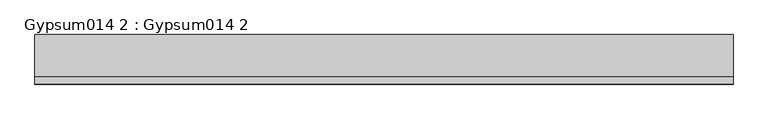
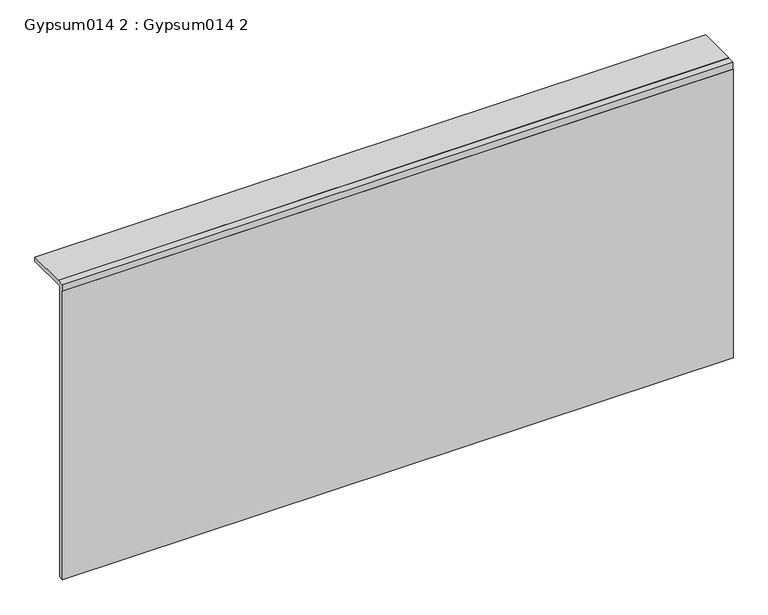
"""IFC4 building model written with IfcOpenShell, lengths in millimetres: proxy geometry, Gypsum014 2 : Gypsum014 2."""

from ifc_helpers import new_model, si_unit, frame, origin, place, context, project, spatial, polyline, outline, extrude, source, transform, mapped, element, save


def gypsum014_2_gypsum014_2_078ccaee(model_context):
    return source(origin(), model_context, "Body", "SweptSolid", [
        extrude(outline(polyline([(9576.3500834, 36582.096), (9576.3500834, 37490.9066598), (9577.6300834, 37490.9066598), (9577.6300834, 37512.0598438), (9598.7832673, 37512.0598438), (9598.7832673, 37513.3398438), (9718.4918386, 37513.3398438), (9718.4918386, 37500.1015625), (9590.6383229, 37500.1015625), (9590.6383229, 36582.096), (9576.3500834, 36582.096)])), frame((3694.2883192, 0.0, 0.0), z_axis=(1.0, 0.0, 0.0), x_axis=(0.0, 1.0, 0.0)), (0.0, 0.0, 1.0), 2000.0),
    ])


if __name__ == "__main__":
    model = new_model("IFC4")
    model_context = context("Model", 3, world=origin())
    ifc_project = project(units=[si_unit("LENGTHUNIT", "METRE", prefix="MILLI")], contexts=[model_context])
    site = spatial("IfcSite", under=ifc_project)
    building = spatial("IfcBuilding", under=site)
    placement = place(None, origin())
    gypsum014_2_gypsum014_2_shape = gypsum014_2_gypsum014_2_078ccaee(model_context)
    element("IfcBuildingElementProxy", 1, Name="Gypsum014 2 : Gypsum014 2", ObjectType="Gypsum014 2 : Gypsum014 2", at=placement, inside=building, context=model_context, shape_type="MappedRepresentation", body=[
        mapped(gypsum014_2_gypsum014_2_shape, transform((0.0, 0.0, 0.0), x_axis=(1.0, 0.0, 0.0), y_axis=(0.0, 1.0, 0.0), z_axis=(0.0, 0.0, 1.0))),
    ])
    save(model, "model.ifc")

# Revit data of these elements
# Type "Gypsum014 2 : Gypsum014 2"
#   NameOverride = "Gypsum014"
# Element 1 (IfcBuildingElementProxy, "Gypsum014 2 : Gypsum014 2")
#   Materials on its faces: "5/8\"  GYPSUM BOARD"
# Materials
#   "5/8\"  GYPSUM BOARD": class "Unassigned", colour RGB 255 255 255, transparency 0, Cost = 0
